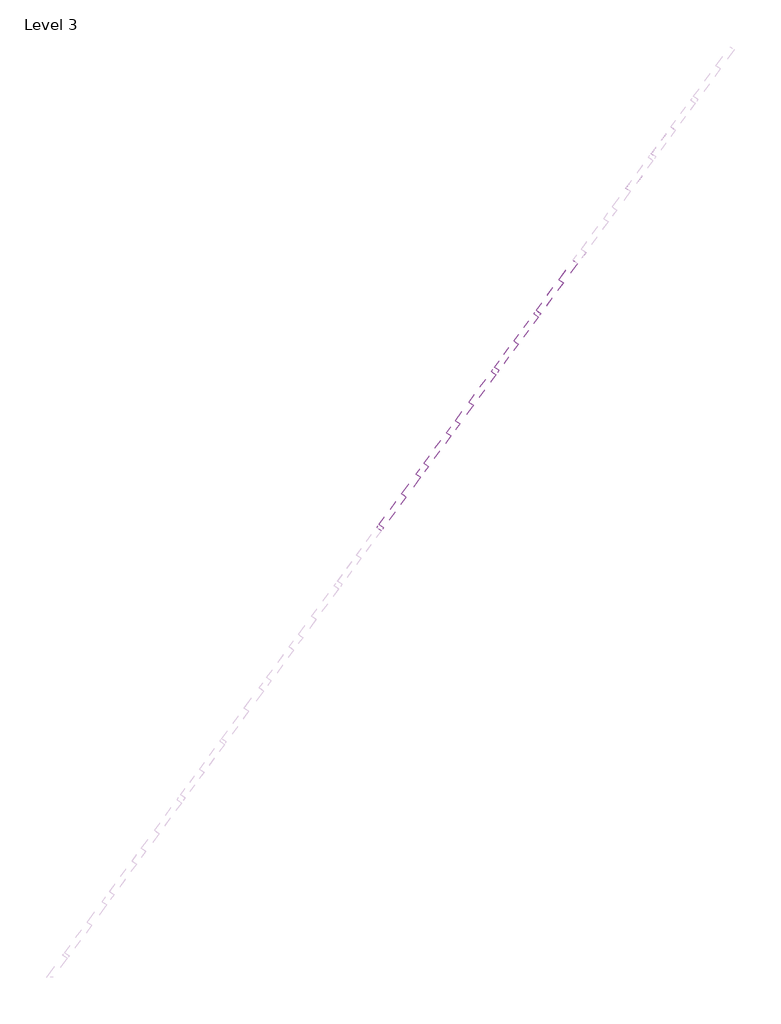
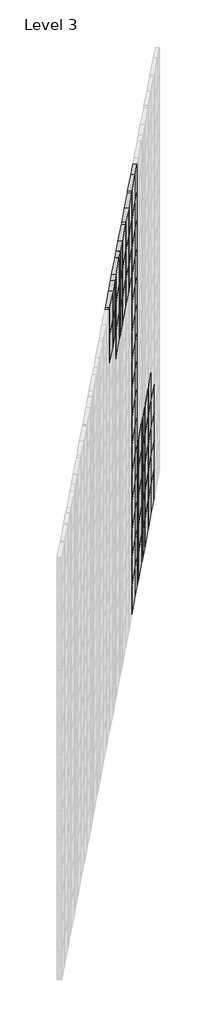
# One storey, part 8 of 9: 117 plates.
"""IFC4 building model written with IfcOpenShell, lengths in millimetres."""

import ifcopenshell
import ifcopenshell.guid

model = None  # the IFC model being written
_history = None  # IfcOwnerHistory: only IFC2X3 demands one
_inside = {}  # id of a spatial element -> (the spatial element, [elements in it])
_under = {}  # id of a project, library or spatial element -> (it, [spatial elements below it])
_declared = {}  # id of a project -> (the project, [libraries it declares])
_typed = {}  # id of a type object -> (the type object, [elements of that type])
_made_of = {}  # id of a material, layer set ... -> (it, [elements and type objects made of it])


def new_model(schema):
    """Start an empty IFC model of exactly this schema.

    Asked for "IFC4X3", IfcOpenShell would pick the latest addendum, in which some entities
    have other attributes; the version numbers below select the first issue.
    IFC2X3 requires an IfcOwnerHistory on every rooted entity: one is made here for all.
    """
    global model, _history
    if schema == "IFC4X3":
        model = ifcopenshell.file(schema_version=(4, 3, 0, 0))
    else:
        model = ifcopenshell.file(schema=schema)
    _inside.clear()
    _under.clear()
    _declared.clear()
    _typed.clear()
    _made_of.clear()
    _history = None
    if model.schema == "IFC2X3":
        org = make("IfcOrganization", Name="unknown")
        user = make(
            "IfcPersonAndOrganization",
            ThePerson=make("IfcPerson", FamilyName="unknown"),
            TheOrganization=org,
        )
        app = make(
            "IfcApplication",
            ApplicationDeveloper=org,
            Version="unknown",
            ApplicationFullName="unknown",
            ApplicationIdentifier="unknown",
        )
        _history = make(
            "IfcOwnerHistory",
            OwningUser=user,
            OwningApplication=app,
            ChangeAction="ADDED",
            CreationDate=0,
        )
    return model


def make(cls, **values):
    """One entity of the class cls with the attributes given. An attribute that is None is left unset."""
    return model.create_entity(
        cls, **{name: value for name, value in values.items() if value is not None}
    )


def rooted(cls, **values):
    """An entity with a GlobalId (a new one), such as an element, a storey or a relation."""
    return make(cls, GlobalId=ifcopenshell.guid.new(), OwnerHistory=_history, **values)


def si_unit(unit_type, name, prefix=None):
    """IfcSIUnit, for example si_unit("LENGTHUNIT", "METRE", prefix="MILLI")."""
    return make("IfcSIUnit", UnitType=unit_type, Prefix=prefix, Name=name)


def assignment(units):
    """IfcUnitAssignment: the units of a project."""
    return None if units is None else make("IfcUnitAssignment", Units=units)


def point(xyz):
    """IfcCartesianPoint."""
    return None if xyz is None else make("IfcCartesianPoint", Coordinates=xyz)


def direction(xyz):
    """IfcDirection."""
    return None if xyz is None else make("IfcDirection", DirectionRatios=xyz)


def frame(location, z_axis=None, x_axis=None):
    """IfcAxis2Placement3D, a coordinate frame: its origin and axes. An axis left out is left unset."""
    return make(
        "IfcAxis2Placement3D",
        Location=point(location),
        Axis=direction(z_axis),
        RefDirection=direction(x_axis),
    )


def origin():
    """The frame at (0, 0, 0) with its axes left unset."""
    return frame((0.0, 0.0, 0.0))


def origin_with_axes():
    """The frame at (0, 0, 0) with the z axis (0, 0, 1) and the x axis (1, 0, 0) written out."""
    return frame((0.0, 0.0, 0.0), z_axis=(0.0, 0.0, 1.0), x_axis=(1.0, 0.0, 0.0))


def place(relative_to, where):
    """IfcLocalPlacement: puts the frame where relative to a parent placement (None: the world)."""
    return make(
        "IfcLocalPlacement", PlacementRelTo=relative_to, RelativePlacement=where
    )


def context(
    kind, dimensions, precision=None, world=None, true_north=None, identifier=None
):
    """IfcGeometricRepresentationContext, for example the 3D "Model" context."""
    return make(
        "IfcGeometricRepresentationContext",
        ContextIdentifier=identifier,
        ContextType=kind,
        CoordinateSpaceDimension=dimensions,
        Precision=precision,
        WorldCoordinateSystem=world,
        TrueNorth=true_north,
    )


def project(units=None, contexts=None):
    """IfcProject with its units and contexts."""
    return rooted(
        "IfcProject",
        Name="project",
        RepresentationContexts=contexts,
        UnitsInContext=assignment(units),
    )


def spatial(cls, under=None, at=None, **own):
    """A site, building, storey or space (cls), placed at a placement, below another one or the project."""
    s = rooted(cls, ObjectPlacement=at, **own)
    if under is not None:
        _under.setdefault(under.id(), (under, []))[1].append(s)
    return s


def polyline(points):
    """IfcPolyline through the points."""
    return make("IfcPolyline", Points=[point(p) for p in points])


def outline(outer, holes=None, kind="AREA"):
    """IfcArbitraryClosedProfileDef: a profile drawn as a closed curve; with holes, ...WithVoids."""
    if holes is None:
        return make("IfcArbitraryClosedProfileDef", ProfileType=kind, OuterCurve=outer)
    return make(
        "IfcArbitraryProfileDefWithVoids",
        ProfileType=kind,
        OuterCurve=outer,
        InnerCurves=holes,
    )


def extrude(swept, where, along, depth):
    """IfcExtrudedAreaSolid: the profile swept, set in the frame where, extruded along a direction by depth."""
    return make(
        "IfcExtrudedAreaSolid",
        SweptArea=swept,
        Position=where,
        ExtrudedDirection=direction(along),
        Depth=depth,
    )


def shape(context_of_items, identifier, shape_type, items):
    """IfcShapeRepresentation: the items that make up one representation, for example the "Body"."""
    return make(
        "IfcShapeRepresentation",
        ContextOfItems=context_of_items,
        RepresentationIdentifier=identifier,
        RepresentationType=shape_type,
        Items=items,
    )


def source(mapping_origin, context_of_items, identifier, shape_type, items):
    """IfcRepresentationMap: a shape defined once, which mapped items show again and again."""
    return make(
        "IfcRepresentationMap",
        MappingOrigin=mapping_origin,
        MappedRepresentation=shape(context_of_items, identifier, shape_type, items),
    )


def transform(
    local_origin,
    x_axis=None,
    y_axis=None,
    z_axis=None,
    scale=None,
    scale2=None,
    scale3=None,
    uniform=True,
):
    """IfcCartesianTransformationOperator3D, or its non-uniform kind. x_axis, y_axis, z_axis: its Axis1, 2, 3."""
    if uniform:
        return make(
            "IfcCartesianTransformationOperator3D",
            Axis1=direction(x_axis),
            Axis2=direction(y_axis),
            LocalOrigin=point(local_origin),
            Scale=scale,
            Axis3=direction(z_axis),
        )
    return make(
        "IfcCartesianTransformationOperator3DnonUniform",
        Axis1=direction(x_axis),
        Axis2=direction(y_axis),
        LocalOrigin=point(local_origin),
        Scale=scale,
        Axis3=direction(z_axis),
        Scale2=scale2,
        Scale3=scale3,
    )


def mapped(mapping_source, mapping_target):
    """IfcMappedItem: shows the shape of a source again, moved by a transform."""
    return make(
        "IfcMappedItem", MappingSource=mapping_source, MappingTarget=mapping_target
    )


def made_of(thing, what):
    """Note that an element or type object is made of a material, layer set ...; save() writes the relation."""
    if what is not None:
        _made_of.setdefault(what.id(), (what, []))[1].append(thing)
    return thing


def element(
    cls,
    number,
    at=None,
    inside=None,
    cuts=None,
    type_object=None,
    material=None,
    context=None,
    identifier="Body",
    shape_type=None,
    held_by="IfcProductDefinitionShape",
    body=None,
    shapes=None,
    **own,
):
    """One element of the class cls, such as IfcWall. Its Tag is "e" and its number.

    at: its placement. inside: the storey or other place that contains it. cuts: it is an
    opening in that element (IfcRelVoidsElement). A single representation is given by context,
    identifier, shape_type and body (its items); several are given by shapes. held_by: the class
    of the entity that holds the representations. save() writes the other relations.
    """
    e = rooted(cls, Tag="e%d" % number, ObjectPlacement=at, **own)
    if body is not None:
        shapes = [shape(context, identifier, shape_type, body)]
    if shapes is not None:
        e.Representation = make(held_by, Representations=shapes)
    if inside is not None:
        _inside.setdefault(inside.id(), (inside, []))[1].append(e)
    if cuts is not None:
        rooted(
            "IfcRelVoidsElement", RelatingBuildingElement=cuts, RelatedOpeningElement=e
        )
    if type_object is not None:
        _typed.setdefault(type_object.id(), (type_object, []))[1].append(e)
    return made_of(e, material)


def aggregate(whole, parts):
    """IfcRelAggregates: a whole, such as a stair, and the parts it consists of."""
    return rooted("IfcRelAggregates", RelatingObject=whole, RelatedObjects=parts)


def save(model, path):
    """Write the relations noted so far, then the file.

    IfcRelAggregates (storeys below a building ...), IfcRelContainedInSpatialStructure (elements
    in a storey), IfcRelDefinesByType, IfcRelAssociatesMaterial and IfcRelDeclares: one each for
    every whole, place, type object, material and project.
    """
    for whole, parts in _under.values():
        aggregate(whole, parts)
    for where, things in _inside.values():
        rooted(
            "IfcRelContainedInSpatialStructure",
            RelatedElements=things,
            RelatingStructure=where,
        )
    for kind, things in _typed.values():
        rooted("IfcRelDefinesByType", RelatedObjects=things, RelatingType=kind)
    for what, things in _made_of.values():
        rooted("IfcRelAssociatesMaterial", RelatedObjects=things, RelatingMaterial=what)
    for by, libraries in _declared.values():
        rooted("IfcRelDeclares", RelatingContext=by, RelatedDefinitions=libraries)
    model.write(path)


def system_panel_glazed_b646d57f(model_context):
    return source(origin(), model_context, "Body", "SweptSolid", [
        extrude(outline(polyline([(8.5363468, 24.5), (-8.5363468, 24.5), (-8.5363468, 49.5), (8.5363468, 49.5), (8.5363468, 24.5)])), origin_with_axes(), (0.0, 0.0, 1.0), 200.0),
    ])


def system_panel_glazed_944c5575(model_context):
    return source(origin(), model_context, "Body", "SweptSolid", [
        extrude(outline(polyline([(30.0531077, 24.5), (-30.0531077, 24.5), (-30.0531077, 49.5), (30.0531077, 49.5), (30.0531077, 24.5)])), origin_with_axes(), (0.0, 0.0, 1.0), 200.0),
    ])


def system_panel_glazed_4b393385(model_context):
    return source(origin(), model_context, "Body", "SweptSolid", [
        extrude(outline(polyline([(51.5698685, 24.5), (-51.5698685, 24.5), (-51.5698685, 49.5), (51.5698685, 49.5), (51.5698685, 24.5)])), origin_with_axes(), (0.0, 0.0, 1.0), 200.0),
    ])


def system_panel_glazed_44cc28f0(model_context):
    return source(origin(), model_context, "Body", "SweptSolid", [
        extrude(outline(polyline([(73.0866293, 24.5), (-73.0866293, 24.5), (-73.0866293, 49.5), (73.0866293, 49.5), (73.0866293, 24.5)])), origin_with_axes(), (0.0, 0.0, 1.0), 200.0),
    ])


def system_panel_glazed_1102e745(model_context):
    return source(origin(), model_context, "Body", "SweptSolid", [
        extrude(outline(polyline([(9.6033902, 24.5), (-9.6033902, 24.5), (-9.6033902, 49.5), (9.6033902, 49.5), (9.6033902, 24.5)])), origin_with_axes(), (0.0, 0.0, 1.0), 200.0),
    ])


def system_panel_glazed_6880485c(model_context):
    return source(origin(), model_context, "Body", "SweptSolid", [
        extrude(outline(polyline([(31.120151, 24.5), (-31.120151, 24.5), (-31.120151, 49.5), (31.120151, 49.5), (31.120151, 24.5)])), origin_with_axes(), (0.0, 0.0, 1.0), 200.0),
    ])


def system_panel_glazed_65218e73(model_context):
    return source(origin(), model_context, "Body", "SweptSolid", [
        extrude(outline(polyline([(52.6369119, 24.5), (-52.6369119, 24.5), (-52.6369119, 49.5), (52.6369119, 49.5), (52.6369119, 24.5)])), origin_with_axes(), (0.0, 0.0, 1.0), 200.0),
    ])


def system_panel_glazed_2ba9a9ff(model_context):
    return source(origin(), model_context, "Body", "SweptSolid", [
        extrude(outline(polyline([(74.1536727, 24.5), (-74.1536727, 24.5), (-74.1536727, 49.5), (74.1536727, 49.5), (74.1536727, 24.5)])), origin_with_axes(), (0.0, 0.0, 1.0), 200.0),
    ])


def system_panel_glazed_87147500(model_context):
    return source(origin(), model_context, "Body", "SweptSolid", [
        extrude(outline(polyline([(10.6704335, 24.5), (-10.6704335, 24.5), (-10.6704335, 49.5), (10.6704335, 49.5), (10.6704335, 24.5)])), origin_with_axes(), (0.0, 0.0, 1.0), 200.0),
    ])


def system_panel_glazed_1ea8d406(model_context):
    return source(origin(), model_context, "Body", "SweptSolid", [
        extrude(outline(polyline([(85.0, 24.5), (-85.0, 24.5), (-85.0, 49.5), (85.0, 49.5), (85.0, 24.5)])), origin_with_axes(), (0.0, 0.0, 1.0), 200.0),
    ])


def system_panel_glazed_a6cffc9f(model_context):
    return source(origin(), model_context, "Body", "SweptSolid", [
        extrude(outline(polyline([(54.9468923, 24.5), (-54.9468923, 24.5), (-54.9468923, 49.5), (54.9468923, 49.5), (54.9468923, 24.5)])), origin_with_axes(), (0.0, 0.0, 1.0), 200.0),
    ])


def system_panel_glazed_52e3984b(model_context):
    return source(origin(), model_context, "Body", "SweptSolid", [
        extrude(outline(polyline([(33.4301315, 24.5), (-33.4301315, 24.5), (-33.4301315, 49.5), (33.4301315, 49.5), (33.4301315, 24.5)])), origin_with_axes(), (0.0, 0.0, 1.0), 200.0),
    ])


def system_panel_glazed_aeb916ba(model_context):
    return source(origin(), model_context, "Body", "SweptSolid", [
        extrude(outline(polyline([(11.9133707, 24.5), (-11.9133707, 24.5), (-11.9133707, 49.5), (11.9133707, 49.5), (11.9133707, 24.5)])), origin_with_axes(), (0.0, 0.0, 1.0), 200.0),
    ])


def system_panel_glazed_a3c9f580(model_context):
    return source(origin(), model_context, "Body", "SweptSolid", [
        extrude(outline(polyline([(75.3966098, 24.5), (-75.3966098, 24.5), (-75.3966098, 49.5), (75.3966098, 49.5), (75.3966098, 24.5)])), origin_with_axes(), (0.0, 0.0, 1.0), 200.0),
    ])


def system_panel_glazed_1c271f2e(model_context):
    return source(origin(), model_context, "Body", "SweptSolid", [
        extrude(outline(polyline([(53.879849, 24.5), (-53.879849, 24.5), (-53.879849, 49.5), (53.879849, 49.5), (53.879849, 24.5)])), origin_with_axes(), (0.0, 0.0, 1.0), 200.0),
    ])


def system_panel_glazed_d23853e5(model_context):
    return source(origin(), model_context, "Body", "SweptSolid", [
        extrude(outline(polyline([(32.3630881, 24.5), (-32.3630881, 24.5), (-32.3630881, 49.5), (32.3630881, 49.5), (32.3630881, 24.5)])), origin_with_axes(), (0.0, 0.0, 1.0), 200.0),
    ])


def system_panel_glazed_c2638314(model_context):
    return source(origin(), model_context, "Body", "SweptSolid", [
        extrude(outline(polyline([(10.8463273, 24.5), (-10.8463273, 24.5), (-10.8463273, 49.5), (10.8463273, 49.5), (10.8463273, 24.5)])), origin_with_axes(), (0.0, 0.0, 1.0), 200.0),
    ])


def system_panel_glazed_937a8ef3(model_context):
    return source(origin(), model_context, "Body", "SweptSolid", [
        extrude(outline(polyline([(74.3295665, 24.5), (-74.3295665, 24.5), (-74.3295665, 49.5), (74.3295665, 49.5), (74.3295665, 24.5)])), origin_with_axes(), (0.0, 0.0, 1.0), 200.0),
    ])


model = new_model("IFC4")

# Units and contexts
model_context = context("Model", 3, world=origin())
ifc_project = project(units=[si_unit("LENGTHUNIT", "METRE", prefix="MILLI")], contexts=[model_context])

# Site, building, storey
site = spatial("IfcSite", under=ifc_project)
building = spatial("IfcBuilding", under=site)
storey = spatial("IfcBuildingStorey", under=building, Name="Level 3", Elevation=22950.0)

# Plates
placement = place(None, origin())
system_panel_glazed_shape = system_panel_glazed_b646d57f(model_context)
element("IfcPlate", 1, ObjectType="System Panel : Glazed", at=placement, inside=storey, context=model_context, shape_type="MappedRepresentation", body=[
    mapped(system_panel_glazed_shape, transform((-31872.965562, 30068.174428, 37700.0), x_axis=(0.5920548138930122, 0.8058976965757569, 0.0), y_axis=(-0.8058976965757569, 0.5920548138930122, 0.0), z_axis=(0.0, 0.0, 1.0))),
])
element("IfcPlate", 2, ObjectType="System Panel : Glazed", at=placement, inside=storey, context=model_context, shape_type="MappedRepresentation", body=[
    mapped(system_panel_glazed_shape, transform((-31872.965562, 30068.174428, 37900.0), x_axis=(0.5920548138930122, 0.8058976965757569, 0.0), y_axis=(-0.8058976965757569, 0.5920548138930122, 0.0), z_axis=(0.0, 0.0, 1.0))),
])
system_panel_glazed_2_shape = system_panel_glazed_944c5575(model_context)
element("IfcPlate", 3, ObjectType="System Panel : Glazed", at=placement, inside=storey, context=model_context, shape_type="MappedRepresentation", body=[
    mapped(system_panel_glazed_2_shape, transform((-31684.4060271, 30324.8393368, 37700.0), x_axis=(0.5920548138930122, 0.8058976965757569, 0.0), y_axis=(-0.8058976965757569, 0.5920548138930122, 0.0), z_axis=(0.0, 0.0, 1.0))),
])
element("IfcPlate", 4, ObjectType="System Panel : Glazed", at=placement, inside=storey, context=model_context, shape_type="MappedRepresentation", body=[
    mapped(system_panel_glazed_2_shape, transform((-31684.4060271, 30324.8393368, 37900.0), x_axis=(0.5920548138930122, 0.8058976965757569, 0.0), y_axis=(-0.8058976965757569, 0.5920548138930122, 0.0), z_axis=(0.0, 0.0, 1.0))),
])
system_panel_glazed_3_shape = system_panel_glazed_4b393385(model_context)
element("IfcPlate", 5, ObjectType="System Panel : Glazed", at=placement, inside=storey, context=model_context, shape_type="MappedRepresentation", body=[
    mapped(system_panel_glazed_3_shape, transform((-31495.8464922, 30581.5042456, 37500.0), x_axis=(0.5920548138930122, 0.8058976965757569, 0.0), y_axis=(-0.8058976965757569, 0.5920548138930122, 0.0), z_axis=(0.0, 0.0, 1.0))),
])
element("IfcPlate", 6, ObjectType="System Panel : Glazed", at=placement, inside=storey, context=model_context, shape_type="MappedRepresentation", body=[
    mapped(system_panel_glazed_3_shape, transform((-31495.8464922, 30581.5042456, 37700.0), x_axis=(0.5920548138930122, 0.8058976965757569, 0.0), y_axis=(-0.8058976965757569, 0.5920548138930122, 0.0), z_axis=(0.0, 0.0, 1.0))),
])
element("IfcPlate", 7, ObjectType="System Panel : Glazed", at=placement, inside=storey, context=model_context, shape_type="MappedRepresentation", body=[
    mapped(system_panel_glazed_3_shape, transform((-31495.8464922, 30581.5042456, 37900.0), x_axis=(0.5920548138930122, 0.8058976965757569, 0.0), y_axis=(-0.8058976965757569, 0.5920548138930122, 0.0), z_axis=(0.0, 0.0, 1.0))),
])
system_panel_glazed_4_shape = system_panel_glazed_44cc28f0(model_context)
element("IfcPlate", 8, ObjectType="System Panel : Glazed", at=placement, inside=storey, context=model_context, shape_type="MappedRepresentation", body=[
    mapped(system_panel_glazed_4_shape, transform((-31307.2869573, 30838.1691545, 37500.0), x_axis=(0.5920548138930122, 0.8058976965757569, 0.0), y_axis=(-0.8058976965757569, 0.5920548138930122, 0.0), z_axis=(0.0, 0.0, 1.0))),
])
element("IfcPlate", 9, ObjectType="System Panel : Glazed", at=placement, inside=storey, context=model_context, shape_type="MappedRepresentation", body=[
    mapped(system_panel_glazed_4_shape, transform((-31307.2869573, 30838.1691545, 37700.0), x_axis=(0.5920548138930122, 0.8058976965757569, 0.0), y_axis=(-0.8058976965757569, 0.5920548138930122, 0.0), z_axis=(0.0, 0.0, 1.0))),
])
element("IfcPlate", 10, ObjectType="System Panel : Glazed", at=placement, inside=storey, context=model_context, shape_type="MappedRepresentation", body=[
    mapped(system_panel_glazed_4_shape, transform((-31307.2869573, 30838.1691545, 37900.0), x_axis=(0.5920548138930122, 0.8058976965757569, 0.0), y_axis=(-0.8058976965757569, 0.5920548138930122, 0.0), z_axis=(0.0, 0.0, 1.0))),
])
system_panel_glazed_5_shape = system_panel_glazed_1102e745(model_context)
element("IfcPlate", 11, ObjectType="System Panel : Glazed", at=placement, inside=storey, context=model_context, shape_type="MappedRepresentation", body=[
    mapped(system_panel_glazed_5_shape, transform((-31169.0520816, 31026.3327591, 35100.0), x_axis=(0.5920548138930122, 0.8058976965757569, 0.0), y_axis=(-0.8058976965757569, 0.5920548138930122, 0.0), z_axis=(0.0, 0.0, 1.0))),
])
element("IfcPlate", 12, ObjectType="System Panel : Glazed", at=placement, inside=storey, context=model_context, shape_type="MappedRepresentation", body=[
    mapped(system_panel_glazed_5_shape, transform((-31169.0520816, 31026.3327591, 35300.0), x_axis=(0.5920548138930122, 0.8058976965757569, 0.0), y_axis=(-0.8058976965757569, 0.5920548138930122, 0.0), z_axis=(0.0, 0.0, 1.0))),
])
element("IfcPlate", 13, ObjectType="System Panel : Glazed", at=placement, inside=storey, context=model_context, shape_type="MappedRepresentation", body=[
    mapped(system_panel_glazed_5_shape, transform((-31169.0520816, 31026.3327591, 35500.0), x_axis=(0.5920548138930122, 0.8058976965757569, 0.0), y_axis=(-0.8058976965757569, 0.5920548138930122, 0.0), z_axis=(0.0, 0.0, 1.0))),
])
element("IfcPlate", 14, ObjectType="System Panel : Glazed", at=placement, inside=storey, context=model_context, shape_type="MappedRepresentation", body=[
    mapped(system_panel_glazed_5_shape, transform((-31169.0520816, 31026.3327591, 35700.0), x_axis=(0.5920548138930122, 0.8058976965757569, 0.0), y_axis=(-0.8058976965757569, 0.5920548138930122, 0.0), z_axis=(0.0, 0.0, 1.0))),
])
element("IfcPlate", 15, ObjectType="System Panel : Glazed", at=placement, inside=storey, context=model_context, shape_type="MappedRepresentation", body=[
    mapped(system_panel_glazed_5_shape, transform((-31169.0520816, 31026.3327591, 35900.0), x_axis=(0.5920548138930122, 0.8058976965757569, 0.0), y_axis=(-0.8058976965757569, 0.5920548138930122, 0.0), z_axis=(0.0, 0.0, 1.0))),
])
element("IfcPlate", 16, ObjectType="System Panel : Glazed", at=placement, inside=storey, context=model_context, shape_type="MappedRepresentation", body=[
    mapped(system_panel_glazed_5_shape, transform((-31169.0520816, 31026.3327591, 36100.0), x_axis=(0.5920548138930122, 0.8058976965757569, 0.0), y_axis=(-0.8058976965757569, 0.5920548138930122, 0.0), z_axis=(0.0, 0.0, 1.0))),
])
element("IfcPlate", 17, ObjectType="System Panel : Glazed", at=placement, inside=storey, context=model_context, shape_type="MappedRepresentation", body=[
    mapped(system_panel_glazed_5_shape, transform((-31169.0520816, 31026.3327591, 36300.0), x_axis=(0.5920548138930122, 0.8058976965757569, 0.0), y_axis=(-0.8058976965757569, 0.5920548138930122, 0.0), z_axis=(0.0, 0.0, 1.0))),
])
element("IfcPlate", 18, ObjectType="System Panel : Glazed", at=placement, inside=storey, context=model_context, shape_type="MappedRepresentation", body=[
    mapped(system_panel_glazed_5_shape, transform((-31169.0520816, 31026.3327591, 36500.0), x_axis=(0.5920548138930122, 0.8058976965757569, 0.0), y_axis=(-0.8058976965757569, 0.5920548138930122, 0.0), z_axis=(0.0, 0.0, 1.0))),
])
element("IfcPlate", 19, ObjectType="System Panel : Glazed", at=placement, inside=storey, context=model_context, shape_type="MappedRepresentation", body=[
    mapped(system_panel_glazed_5_shape, transform((-31169.0520816, 31026.3327591, 36700.0), x_axis=(0.5920548138930122, 0.8058976965757569, 0.0), y_axis=(-0.8058976965757569, 0.5920548138930122, 0.0), z_axis=(0.0, 0.0, 1.0))),
])
element("IfcPlate", 20, ObjectType="System Panel : Glazed", at=placement, inside=storey, context=model_context, shape_type="MappedRepresentation", body=[
    mapped(system_panel_glazed_5_shape, transform((-31169.0520816, 31026.3327591, 36900.0), x_axis=(0.5920548138930122, 0.8058976965757569, 0.0), y_axis=(-0.8058976965757569, 0.5920548138930122, 0.0), z_axis=(0.0, 0.0, 1.0))),
])
element("IfcPlate", 21, ObjectType="System Panel : Glazed", at=placement, inside=storey, context=model_context, shape_type="MappedRepresentation", body=[
    mapped(system_panel_glazed_5_shape, transform((-31169.0520816, 31026.3327591, 37100.0), x_axis=(0.5920548138930122, 0.8058976965757569, 0.0), y_axis=(-0.8058976965757569, 0.5920548138930122, 0.0), z_axis=(0.0, 0.0, 1.0))),
])
element("IfcPlate", 22, ObjectType="System Panel : Glazed", at=placement, inside=storey, context=model_context, shape_type="MappedRepresentation", body=[
    mapped(system_panel_glazed_5_shape, transform((-31169.0520816, 31026.3327591, 37300.0), x_axis=(0.5920548138930122, 0.8058976965757569, 0.0), y_axis=(-0.8058976965757569, 0.5920548138930122, 0.0), z_axis=(0.0, 0.0, 1.0))),
])
element("IfcPlate", 23, ObjectType="System Panel : Glazed", at=placement, inside=storey, context=model_context, shape_type="MappedRepresentation", body=[
    mapped(system_panel_glazed_5_shape, transform((-31169.0520816, 31026.3327591, 37500.0), x_axis=(0.5920548138930122, 0.8058976965757569, 0.0), y_axis=(-0.8058976965757569, 0.5920548138930122, 0.0), z_axis=(0.0, 0.0, 1.0))),
])
element("IfcPlate", 24, ObjectType="System Panel : Glazed", at=placement, inside=storey, context=model_context, shape_type="MappedRepresentation", body=[
    mapped(system_panel_glazed_5_shape, transform((-31169.0520816, 31026.3327591, 37700.0), x_axis=(0.5920548138930122, 0.8058976965757569, 0.0), y_axis=(-0.8058976965757569, 0.5920548138930122, 0.0), z_axis=(0.0, 0.0, 1.0))),
])
element("IfcPlate", 25, ObjectType="System Panel : Glazed", at=placement, inside=storey, context=model_context, shape_type="MappedRepresentation", body=[
    mapped(system_panel_glazed_5_shape, transform((-31169.0520816, 31026.3327591, 37900.0), x_axis=(0.5920548138930122, 0.8058976965757569, 0.0), y_axis=(-0.8058976965757569, 0.5920548138930122, 0.0), z_axis=(0.0, 0.0, 1.0))),
])
system_panel_glazed_6_shape = system_panel_glazed_6880485c(model_context)
element("IfcPlate", 26, ObjectType="System Panel : Glazed", at=placement, inside=storey, context=model_context, shape_type="MappedRepresentation", body=[
    mapped(system_panel_glazed_6_shape, transform((-30980.4925467, 31282.997668, 35100.0), x_axis=(0.5920548138930122, 0.8058976965757569, 0.0), y_axis=(-0.8058976965757569, 0.5920548138930122, 0.0), z_axis=(0.0, 0.0, 1.0))),
])
element("IfcPlate", 27, ObjectType="System Panel : Glazed", at=placement, inside=storey, context=model_context, shape_type="MappedRepresentation", body=[
    mapped(system_panel_glazed_6_shape, transform((-30980.4925467, 31282.997668, 35300.0), x_axis=(0.5920548138930122, 0.8058976965757569, 0.0), y_axis=(-0.8058976965757569, 0.5920548138930122, 0.0), z_axis=(0.0, 0.0, 1.0))),
])
element("IfcPlate", 28, ObjectType="System Panel : Glazed", at=placement, inside=storey, context=model_context, shape_type="MappedRepresentation", body=[
    mapped(system_panel_glazed_6_shape, transform((-30980.4925467, 31282.997668, 35500.0), x_axis=(0.5920548138930122, 0.8058976965757569, 0.0), y_axis=(-0.8058976965757569, 0.5920548138930122, 0.0), z_axis=(0.0, 0.0, 1.0))),
])
element("IfcPlate", 29, ObjectType="System Panel : Glazed", at=placement, inside=storey, context=model_context, shape_type="MappedRepresentation", body=[
    mapped(system_panel_glazed_6_shape, transform((-30980.4925467, 31282.997668, 35700.0), x_axis=(0.5920548138930122, 0.8058976965757569, 0.0), y_axis=(-0.8058976965757569, 0.5920548138930122, 0.0), z_axis=(0.0, 0.0, 1.0))),
])
element("IfcPlate", 30, ObjectType="System Panel : Glazed", at=placement, inside=storey, context=model_context, shape_type="MappedRepresentation", body=[
    mapped(system_panel_glazed_6_shape, transform((-30980.4925467, 31282.997668, 35900.0), x_axis=(0.5920548138930122, 0.8058976965757569, 0.0), y_axis=(-0.8058976965757569, 0.5920548138930122, 0.0), z_axis=(0.0, 0.0, 1.0))),
])
system_panel_glazed_7_shape = system_panel_glazed_65218e73(model_context)
element("IfcPlate", 31, ObjectType="System Panel : Glazed", at=placement, inside=storey, context=model_context, shape_type="MappedRepresentation", body=[
    mapped(system_panel_glazed_7_shape, transform((-30791.9330118, 31539.6625768, 35100.0), x_axis=(0.5920548138930122, 0.8058976965757569, 0.0), y_axis=(-0.8058976965757569, 0.5920548138930122, 0.0), z_axis=(0.0, 0.0, 1.0))),
])
element("IfcPlate", 32, ObjectType="System Panel : Glazed", at=placement, inside=storey, context=model_context, shape_type="MappedRepresentation", body=[
    mapped(system_panel_glazed_7_shape, transform((-30791.9330118, 31539.6625768, 35300.0), x_axis=(0.5920548138930122, 0.8058976965757569, 0.0), y_axis=(-0.8058976965757569, 0.5920548138930122, 0.0), z_axis=(0.0, 0.0, 1.0))),
])
element("IfcPlate", 33, ObjectType="System Panel : Glazed", at=placement, inside=storey, context=model_context, shape_type="MappedRepresentation", body=[
    mapped(system_panel_glazed_7_shape, transform((-30791.9330118, 31539.6625768, 35500.0), x_axis=(0.5920548138930122, 0.8058976965757569, 0.0), y_axis=(-0.8058976965757569, 0.5920548138930122, 0.0), z_axis=(0.0, 0.0, 1.0))),
])
element("IfcPlate", 34, ObjectType="System Panel : Glazed", at=placement, inside=storey, context=model_context, shape_type="MappedRepresentation", body=[
    mapped(system_panel_glazed_7_shape, transform((-30791.9330118, 31539.6625768, 35700.0), x_axis=(0.5920548138930122, 0.8058976965757569, 0.0), y_axis=(-0.8058976965757569, 0.5920548138930122, 0.0), z_axis=(0.0, 0.0, 1.0))),
])
element("IfcPlate", 35, ObjectType="System Panel : Glazed", at=placement, inside=storey, context=model_context, shape_type="MappedRepresentation", body=[
    mapped(system_panel_glazed_7_shape, transform((-30791.9330118, 31539.6625768, 35900.0), x_axis=(0.5920548138930122, 0.8058976965757569, 0.0), y_axis=(-0.8058976965757569, 0.5920548138930122, 0.0), z_axis=(0.0, 0.0, 1.0))),
])
system_panel_glazed_8_shape = system_panel_glazed_2ba9a9ff(model_context)
element("IfcPlate", 36, ObjectType="System Panel : Glazed", at=placement, inside=storey, context=model_context, shape_type="MappedRepresentation", body=[
    mapped(system_panel_glazed_8_shape, transform((-30603.373477, 31796.3274856, 35100.0), x_axis=(0.5920548138930122, 0.8058976965757569, 0.0), y_axis=(-0.8058976965757569, 0.5920548138930122, 0.0), z_axis=(0.0, 0.0, 1.0))),
])
element("IfcPlate", 37, ObjectType="System Panel : Glazed", at=placement, inside=storey, context=model_context, shape_type="MappedRepresentation", body=[
    mapped(system_panel_glazed_8_shape, transform((-30603.373477, 31796.3274856, 35300.0), x_axis=(0.5920548138930122, 0.8058976965757569, 0.0), y_axis=(-0.8058976965757569, 0.5920548138930122, 0.0), z_axis=(0.0, 0.0, 1.0))),
])
element("IfcPlate", 38, ObjectType="System Panel : Glazed", at=placement, inside=storey, context=model_context, shape_type="MappedRepresentation", body=[
    mapped(system_panel_glazed_8_shape, transform((-30603.373477, 31796.3274856, 35500.0), x_axis=(0.5920548138930122, 0.8058976965757569, 0.0), y_axis=(-0.8058976965757569, 0.5920548138930122, 0.0), z_axis=(0.0, 0.0, 1.0))),
])
element("IfcPlate", 39, ObjectType="System Panel : Glazed", at=placement, inside=storey, context=model_context, shape_type="MappedRepresentation", body=[
    mapped(system_panel_glazed_8_shape, transform((-30603.373477, 31796.3274856, 35700.0), x_axis=(0.5920548138930122, 0.8058976965757569, 0.0), y_axis=(-0.8058976965757569, 0.5920548138930122, 0.0), z_axis=(0.0, 0.0, 1.0))),
])
element("IfcPlate", 40, ObjectType="System Panel : Glazed", at=placement, inside=storey, context=model_context, shape_type="MappedRepresentation", body=[
    mapped(system_panel_glazed_8_shape, transform((-30603.373477, 31796.3274856, 35900.0), x_axis=(0.5920548138930122, 0.8058976965757569, 0.0), y_axis=(-0.8058976965757569, 0.5920548138930122, 0.0), z_axis=(0.0, 0.0, 1.0))),
])
system_panel_glazed_9_shape = system_panel_glazed_87147500(model_context)
element("IfcPlate", 41, ObjectType="System Panel : Glazed", at=placement, inside=storey, context=model_context, shape_type="MappedRepresentation", body=[
    mapped(system_panel_glazed_9_shape, transform((-30465.1386012, 31984.4910903, 35100.0), x_axis=(0.5920548138930122, 0.8058976965757569, 0.0), y_axis=(-0.8058976965757569, 0.5920548138930122, 0.0), z_axis=(0.0, 0.0, 1.0))),
])
element("IfcPlate", 42, ObjectType="System Panel : Glazed", at=placement, inside=storey, context=model_context, shape_type="MappedRepresentation", body=[
    mapped(system_panel_glazed_9_shape, transform((-30465.1386012, 31984.4910903, 35300.0), x_axis=(0.5920548138930122, 0.8058976965757569, 0.0), y_axis=(-0.8058976965757569, 0.5920548138930122, 0.0), z_axis=(0.0, 0.0, 1.0))),
])
element("IfcPlate", 43, ObjectType="System Panel : Glazed", at=placement, inside=storey, context=model_context, shape_type="MappedRepresentation", body=[
    mapped(system_panel_glazed_9_shape, transform((-30465.1386012, 31984.4910903, 35500.0), x_axis=(0.5920548138930122, 0.8058976965757569, 0.0), y_axis=(-0.8058976965757569, 0.5920548138930122, 0.0), z_axis=(0.0, 0.0, 1.0))),
])
element("IfcPlate", 44, ObjectType="System Panel : Glazed", at=placement, inside=storey, context=model_context, shape_type="MappedRepresentation", body=[
    mapped(system_panel_glazed_9_shape, transform((-30465.1386012, 31984.4910903, 35700.0), x_axis=(0.5920548138930122, 0.8058976965757569, 0.0), y_axis=(-0.8058976965757569, 0.5920548138930122, 0.0), z_axis=(0.0, 0.0, 1.0))),
])
system_panel_glazed_10_shape = system_panel_glazed_1ea8d406(model_context)
element("IfcPlate", 45, ObjectType="System Panel : Glazed", at=placement, inside=storey, context=model_context, shape_type="MappedRepresentation", body=[
    mapped(system_panel_glazed_10_shape, transform((-31113.0416891, 31102.5734133, 35100.0), x_axis=(0.5920548138930122, 0.8058976965757569, 0.0), y_axis=(-0.8058976965757569, 0.5920548138930122, 0.0), z_axis=(0.0, 0.0, 1.0))),
])
element("IfcPlate", 46, ObjectType="System Panel : Glazed", at=placement, inside=storey, context=model_context, shape_type="MappedRepresentation", body=[
    mapped(system_panel_glazed_10_shape, transform((-30911.7430523, 31376.5786302, 35100.0), x_axis=(0.5920548138930122, 0.8058976965757569, 0.0), y_axis=(-0.8058976965757569, 0.5920548138930122, 0.0), z_axis=(0.0, 0.0, 1.0))),
])
element("IfcPlate", 47, ObjectType="System Panel : Glazed", at=placement, inside=storey, context=model_context, shape_type="MappedRepresentation", body=[
    mapped(system_panel_glazed_10_shape, transform((-30710.4444156, 31650.583847, 35100.0), x_axis=(0.5920548138930122, 0.8058976965757569, 0.0), y_axis=(-0.8058976965757569, 0.5920548138930122, 0.0), z_axis=(0.0, 0.0, 1.0))),
])
element("IfcPlate", 48, ObjectType="System Panel : Glazed", at=placement, inside=storey, context=model_context, shape_type="MappedRepresentation", body=[
    mapped(system_panel_glazed_10_shape, transform((-31113.0416891, 31102.5734133, 35300.0), x_axis=(0.5920548138930122, 0.8058976965757569, 0.0), y_axis=(-0.8058976965757569, 0.5920548138930122, 0.0), z_axis=(0.0, 0.0, 1.0))),
])
element("IfcPlate", 49, ObjectType="System Panel : Glazed", at=placement, inside=storey, context=model_context, shape_type="MappedRepresentation", body=[
    mapped(system_panel_glazed_10_shape, transform((-30911.7430523, 31376.5786302, 35300.0), x_axis=(0.5920548138930122, 0.8058976965757569, 0.0), y_axis=(-0.8058976965757569, 0.5920548138930122, 0.0), z_axis=(0.0, 0.0, 1.0))),
])
element("IfcPlate", 50, ObjectType="System Panel : Glazed", at=placement, inside=storey, context=model_context, shape_type="MappedRepresentation", body=[
    mapped(system_panel_glazed_10_shape, transform((-30710.4444156, 31650.583847, 35300.0), x_axis=(0.5920548138930122, 0.8058976965757569, 0.0), y_axis=(-0.8058976965757569, 0.5920548138930122, 0.0), z_axis=(0.0, 0.0, 1.0))),
])
element("IfcPlate", 51, ObjectType="System Panel : Glazed", at=placement, inside=storey, context=model_context, shape_type="MappedRepresentation", body=[
    mapped(system_panel_glazed_10_shape, transform((-31113.0416891, 31102.5734133, 35500.0), x_axis=(0.5920548138930122, 0.8058976965757569, 0.0), y_axis=(-0.8058976965757569, 0.5920548138930122, 0.0), z_axis=(0.0, 0.0, 1.0))),
])
element("IfcPlate", 52, ObjectType="System Panel : Glazed", at=placement, inside=storey, context=model_context, shape_type="MappedRepresentation", body=[
    mapped(system_panel_glazed_10_shape, transform((-30911.7430523, 31376.5786302, 35500.0), x_axis=(0.5920548138930122, 0.8058976965757569, 0.0), y_axis=(-0.8058976965757569, 0.5920548138930122, 0.0), z_axis=(0.0, 0.0, 1.0))),
])
element("IfcPlate", 53, ObjectType="System Panel : Glazed", at=placement, inside=storey, context=model_context, shape_type="MappedRepresentation", body=[
    mapped(system_panel_glazed_10_shape, transform((-30710.4444156, 31650.583847, 35500.0), x_axis=(0.5920548138930122, 0.8058976965757569, 0.0), y_axis=(-0.8058976965757569, 0.5920548138930122, 0.0), z_axis=(0.0, 0.0, 1.0))),
])
element("IfcPlate", 54, ObjectType="System Panel : Glazed", at=placement, inside=storey, context=model_context, shape_type="MappedRepresentation", body=[
    mapped(system_panel_glazed_10_shape, transform((-31113.0416891, 31102.5734133, 35700.0), x_axis=(0.5920548138930122, 0.8058976965757569, 0.0), y_axis=(-0.8058976965757569, 0.5920548138930122, 0.0), z_axis=(0.0, 0.0, 1.0))),
])
element("IfcPlate", 55, ObjectType="System Panel : Glazed", at=placement, inside=storey, context=model_context, shape_type="MappedRepresentation", body=[
    mapped(system_panel_glazed_10_shape, transform((-30911.7430523, 31376.5786302, 35700.0), x_axis=(0.5920548138930122, 0.8058976965757569, 0.0), y_axis=(-0.8058976965757569, 0.5920548138930122, 0.0), z_axis=(0.0, 0.0, 1.0))),
])
element("IfcPlate", 56, ObjectType="System Panel : Glazed", at=placement, inside=storey, context=model_context, shape_type="MappedRepresentation", body=[
    mapped(system_panel_glazed_10_shape, transform((-30710.4444156, 31650.583847, 35700.0), x_axis=(0.5920548138930122, 0.8058976965757569, 0.0), y_axis=(-0.8058976965757569, 0.5920548138930122, 0.0), z_axis=(0.0, 0.0, 1.0))),
])
element("IfcPlate", 57, ObjectType="System Panel : Glazed", at=placement, inside=storey, context=model_context, shape_type="MappedRepresentation", body=[
    mapped(system_panel_glazed_10_shape, transform((-31113.0416891, 31102.5734133, 35900.0), x_axis=(0.5920548138930122, 0.8058976965757569, 0.0), y_axis=(-0.8058976965757569, 0.5920548138930122, 0.0), z_axis=(0.0, 0.0, 1.0))),
])
element("IfcPlate", 58, ObjectType="System Panel : Glazed", at=placement, inside=storey, context=model_context, shape_type="MappedRepresentation", body=[
    mapped(system_panel_glazed_10_shape, transform((-30911.7430523, 31376.5786302, 35900.0), x_axis=(0.5920548138930122, 0.8058976965757569, 0.0), y_axis=(-0.8058976965757569, 0.5920548138930122, 0.0), z_axis=(0.0, 0.0, 1.0))),
])
element("IfcPlate", 59, ObjectType="System Panel : Glazed", at=placement, inside=storey, context=model_context, shape_type="MappedRepresentation", body=[
    mapped(system_panel_glazed_10_shape, transform((-30710.4444156, 31650.583847, 35900.0), x_axis=(0.5920548138930122, 0.8058976965757569, 0.0), y_axis=(-0.8058976965757569, 0.5920548138930122, 0.0), z_axis=(0.0, 0.0, 1.0))),
])
element("IfcPlate", 60, ObjectType="System Panel : Glazed", at=placement, inside=storey, context=model_context, shape_type="MappedRepresentation", body=[
    mapped(system_panel_glazed_10_shape, transform((-31113.0416891, 31102.5734133, 36100.0), x_axis=(0.5920548138930122, 0.8058976965757569, 0.0), y_axis=(-0.8058976965757569, 0.5920548138930122, 0.0), z_axis=(0.0, 0.0, 1.0))),
])
element("IfcPlate", 61, ObjectType="System Panel : Glazed", at=placement, inside=storey, context=model_context, shape_type="MappedRepresentation", body=[
    mapped(system_panel_glazed_10_shape, transform((-31113.0416891, 31102.5734133, 36300.0), x_axis=(0.5920548138930122, 0.8058976965757569, 0.0), y_axis=(-0.8058976965757569, 0.5920548138930122, 0.0), z_axis=(0.0, 0.0, 1.0))),
])
element("IfcPlate", 62, ObjectType="System Panel : Glazed", at=placement, inside=storey, context=model_context, shape_type="MappedRepresentation", body=[
    mapped(system_panel_glazed_10_shape, transform((-31113.0416891, 31102.5734133, 36500.0), x_axis=(0.5920548138930122, 0.8058976965757569, 0.0), y_axis=(-0.8058976965757569, 0.5920548138930122, 0.0), z_axis=(0.0, 0.0, 1.0))),
])
element("IfcPlate", 63, ObjectType="System Panel : Glazed", at=placement, inside=storey, context=model_context, shape_type="MappedRepresentation", body=[
    mapped(system_panel_glazed_10_shape, transform((-31113.0416891, 31102.5734133, 36700.0), x_axis=(0.5920548138930122, 0.8058976965757569, 0.0), y_axis=(-0.8058976965757569, 0.5920548138930122, 0.0), z_axis=(0.0, 0.0, 1.0))),
])
element("IfcPlate", 64, ObjectType="System Panel : Glazed", at=placement, inside=storey, context=model_context, shape_type="MappedRepresentation", body=[
    mapped(system_panel_glazed_10_shape, transform((-31113.0416891, 31102.5734133, 36900.0), x_axis=(0.5920548138930122, 0.8058976965757569, 0.0), y_axis=(-0.8058976965757569, 0.5920548138930122, 0.0), z_axis=(0.0, 0.0, 1.0))),
])
element("IfcPlate", 65, ObjectType="System Panel : Glazed", at=placement, inside=storey, context=model_context, shape_type="MappedRepresentation", body=[
    mapped(system_panel_glazed_10_shape, transform((-31113.0416891, 31102.5734133, 37100.0), x_axis=(0.5920548138930122, 0.8058976965757569, 0.0), y_axis=(-0.8058976965757569, 0.5920548138930122, 0.0), z_axis=(0.0, 0.0, 1.0))),
])
element("IfcPlate", 66, ObjectType="System Panel : Glazed", at=placement, inside=storey, context=model_context, shape_type="MappedRepresentation", body=[
    mapped(system_panel_glazed_10_shape, transform((-31113.0416891, 31102.5734133, 37300.0), x_axis=(0.5920548138930122, 0.8058976965757569, 0.0), y_axis=(-0.8058976965757569, 0.5920548138930122, 0.0), z_axis=(0.0, 0.0, 1.0))),
])
element("IfcPlate", 67, ObjectType="System Panel : Glazed", at=placement, inside=storey, context=model_context, shape_type="MappedRepresentation", body=[
    mapped(system_panel_glazed_10_shape, transform((-31616.2882809, 30417.5603713, 37500.0), x_axis=(0.5920548138930122, 0.8058976965757569, 0.0), y_axis=(-0.8058976965757569, 0.5920548138930122, 0.0), z_axis=(0.0, 0.0, 1.0))),
])
element("IfcPlate", 68, ObjectType="System Panel : Glazed", at=placement, inside=storey, context=model_context, shape_type="MappedRepresentation", body=[
    mapped(system_panel_glazed_10_shape, transform((-31414.9896441, 30691.5655881, 37500.0), x_axis=(0.5920548138930122, 0.8058976965757569, 0.0), y_axis=(-0.8058976965757569, 0.5920548138930122, 0.0), z_axis=(0.0, 0.0, 1.0))),
])
element("IfcPlate", 69, ObjectType="System Panel : Glazed", at=placement, inside=storey, context=model_context, shape_type="MappedRepresentation", body=[
    mapped(system_panel_glazed_10_shape, transform((-31113.0416891, 31102.5734133, 37500.0), x_axis=(0.5920548138930122, 0.8058976965757569, 0.0), y_axis=(-0.8058976965757569, 0.5920548138930122, 0.0), z_axis=(0.0, 0.0, 1.0))),
])
element("IfcPlate", 70, ObjectType="System Panel : Glazed", at=placement, inside=storey, context=model_context, shape_type="MappedRepresentation", body=[
    mapped(system_panel_glazed_10_shape, transform((-31817.5869176, 30143.5551544, 37700.0), x_axis=(0.5920548138930122, 0.8058976965757569, 0.0), y_axis=(-0.8058976965757569, 0.5920548138930122, 0.0), z_axis=(0.0, 0.0, 1.0))),
])
element("IfcPlate", 71, ObjectType="System Panel : Glazed", at=placement, inside=storey, context=model_context, shape_type="MappedRepresentation", body=[
    mapped(system_panel_glazed_10_shape, transform((-31616.2882809, 30417.5603713, 37700.0), x_axis=(0.5920548138930122, 0.8058976965757569, 0.0), y_axis=(-0.8058976965757569, 0.5920548138930122, 0.0), z_axis=(0.0, 0.0, 1.0))),
])
element("IfcPlate", 72, ObjectType="System Panel : Glazed", at=placement, inside=storey, context=model_context, shape_type="MappedRepresentation", body=[
    mapped(system_panel_glazed_10_shape, transform((-31414.9896441, 30691.5655881, 37700.0), x_axis=(0.5920548138930122, 0.8058976965757569, 0.0), y_axis=(-0.8058976965757569, 0.5920548138930122, 0.0), z_axis=(0.0, 0.0, 1.0))),
])
element("IfcPlate", 73, ObjectType="System Panel : Glazed", at=placement, inside=storey, context=model_context, shape_type="MappedRepresentation", body=[
    mapped(system_panel_glazed_10_shape, transform((-31113.0416891, 31102.5734133, 37700.0), x_axis=(0.5920548138930122, 0.8058976965757569, 0.0), y_axis=(-0.8058976965757569, 0.5920548138930122, 0.0), z_axis=(0.0, 0.0, 1.0))),
])
element("IfcPlate", 74, ObjectType="System Panel : Glazed", at=placement, inside=storey, context=model_context, shape_type="MappedRepresentation", body=[
    mapped(system_panel_glazed_10_shape, transform((-31817.5869176, 30143.5551544, 37900.0), x_axis=(0.5920548138930122, 0.8058976965757569, 0.0), y_axis=(-0.8058976965757569, 0.5920548138930122, 0.0), z_axis=(0.0, 0.0, 1.0))),
])
element("IfcPlate", 75, ObjectType="System Panel : Glazed", at=placement, inside=storey, context=model_context, shape_type="MappedRepresentation", body=[
    mapped(system_panel_glazed_10_shape, transform((-31616.2882809, 30417.5603713, 37900.0), x_axis=(0.5920548138930122, 0.8058976965757569, 0.0), y_axis=(-0.8058976965757569, 0.5920548138930122, 0.0), z_axis=(0.0, 0.0, 1.0))),
])
element("IfcPlate", 76, ObjectType="System Panel : Glazed", at=placement, inside=storey, context=model_context, shape_type="MappedRepresentation", body=[
    mapped(system_panel_glazed_10_shape, transform((-31414.9896441, 30691.5655881, 37900.0), x_axis=(0.5920548138930122, 0.8058976965757569, 0.0), y_axis=(-0.8058976965757569, 0.5920548138930122, 0.0), z_axis=(0.0, 0.0, 1.0))),
])
element("IfcPlate", 77, ObjectType="System Panel : Glazed", at=placement, inside=storey, context=model_context, shape_type="MappedRepresentation", body=[
    mapped(system_panel_glazed_10_shape, transform((-31113.0416891, 31102.5734133, 37900.0), x_axis=(0.5920548138930122, 0.8058976965757569, 0.0), y_axis=(-0.8058976965757569, 0.5920548138930122, 0.0), z_axis=(0.0, 0.0, 1.0))),
])
system_panel_glazed_11_shape = system_panel_glazed_a6cffc9f(model_context)
element("IfcPlate", 78, ObjectType="System Panel : Glazed", at=placement, inside=storey, context=model_context, shape_type="MappedRepresentation", body=[
    mapped(system_panel_glazed_11_shape, transform((-31734.7306863, 30256.3380326, 37700.0), x_axis=(0.5920548138930122, 0.8058976965757569, 0.0), y_axis=(-0.8058976965757569, 0.5920548138930122, 0.0), z_axis=(0.0, 0.0, 1.0))),
])
element("IfcPlate", 79, ObjectType="System Panel : Glazed", at=placement, inside=storey, context=model_context, shape_type="MappedRepresentation", body=[
    mapped(system_panel_glazed_11_shape, transform((-31734.7306863, 30256.3380326, 37900.0), x_axis=(0.5920548138930122, 0.8058976965757569, 0.0), y_axis=(-0.8058976965757569, 0.5920548138930122, 0.0), z_axis=(0.0, 0.0, 1.0))),
])
system_panel_glazed_12_shape = system_panel_glazed_52e3984b(model_context)
element("IfcPlate", 80, ObjectType="System Panel : Glazed", at=placement, inside=storey, context=model_context, shape_type="MappedRepresentation", body=[
    mapped(system_panel_glazed_12_shape, transform((-31546.1711514, 30513.0029414, 37500.0), x_axis=(0.5920548138930122, 0.8058976965757569, 0.0), y_axis=(-0.8058976965757569, 0.5920548138930122, 0.0), z_axis=(0.0, 0.0, 1.0))),
])
element("IfcPlate", 81, ObjectType="System Panel : Glazed", at=placement, inside=storey, context=model_context, shape_type="MappedRepresentation", body=[
    mapped(system_panel_glazed_12_shape, transform((-31546.1711514, 30513.0029414, 37700.0), x_axis=(0.5920548138930122, 0.8058976965757569, 0.0), y_axis=(-0.8058976965757569, 0.5920548138930122, 0.0), z_axis=(0.0, 0.0, 1.0))),
])
element("IfcPlate", 82, ObjectType="System Panel : Glazed", at=placement, inside=storey, context=model_context, shape_type="MappedRepresentation", body=[
    mapped(system_panel_glazed_12_shape, transform((-31546.1711514, 30513.0029414, 37900.0), x_axis=(0.5920548138930122, 0.8058976965757569, 0.0), y_axis=(-0.8058976965757569, 0.5920548138930122, 0.0), z_axis=(0.0, 0.0, 1.0))),
])
system_panel_glazed_13_shape = system_panel_glazed_aeb916ba(model_context)
element("IfcPlate", 83, ObjectType="System Panel : Glazed", at=placement, inside=storey, context=model_context, shape_type="MappedRepresentation", body=[
    mapped(system_panel_glazed_13_shape, transform((-31357.6116165, 30769.6678503, 37500.0), x_axis=(0.5920548138930122, 0.8058976965757569, 0.0), y_axis=(-0.8058976965757569, 0.5920548138930122, 0.0), z_axis=(0.0, 0.0, 1.0))),
])
element("IfcPlate", 84, ObjectType="System Panel : Glazed", at=placement, inside=storey, context=model_context, shape_type="MappedRepresentation", body=[
    mapped(system_panel_glazed_13_shape, transform((-31357.6116165, 30769.6678503, 37700.0), x_axis=(0.5920548138930122, 0.8058976965757569, 0.0), y_axis=(-0.8058976965757569, 0.5920548138930122, 0.0), z_axis=(0.0, 0.0, 1.0))),
])
element("IfcPlate", 85, ObjectType="System Panel : Glazed", at=placement, inside=storey, context=model_context, shape_type="MappedRepresentation", body=[
    mapped(system_panel_glazed_13_shape, transform((-31357.6116165, 30769.6678503, 37900.0), x_axis=(0.5920548138930122, 0.8058976965757569, 0.0), y_axis=(-0.8058976965757569, 0.5920548138930122, 0.0), z_axis=(0.0, 0.0, 1.0))),
])
system_panel_glazed_14_shape = system_panel_glazed_a3c9f580(model_context)
element("IfcPlate", 86, ObjectType="System Panel : Glazed", at=placement, inside=storey, context=model_context, shape_type="MappedRepresentation", body=[
    mapped(system_panel_glazed_14_shape, transform((-31219.3767408, 30957.8314549, 37500.0), x_axis=(0.5920548138930122, 0.8058976965757569, 0.0), y_axis=(-0.8058976965757569, 0.5920548138930122, 0.0), z_axis=(0.0, 0.0, 1.0))),
])
element("IfcPlate", 87, ObjectType="System Panel : Glazed", at=placement, inside=storey, context=model_context, shape_type="MappedRepresentation", body=[
    mapped(system_panel_glazed_14_shape, transform((-31219.3767408, 30957.8314549, 37700.0), x_axis=(0.5920548138930122, 0.8058976965757569, 0.0), y_axis=(-0.8058976965757569, 0.5920548138930122, 0.0), z_axis=(0.0, 0.0, 1.0))),
])
element("IfcPlate", 88, ObjectType="System Panel : Glazed", at=placement, inside=storey, context=model_context, shape_type="MappedRepresentation", body=[
    mapped(system_panel_glazed_14_shape, transform((-31219.3767408, 30957.8314549, 37900.0), x_axis=(0.5920548138930122, 0.8058976965757569, 0.0), y_axis=(-0.8058976965757569, 0.5920548138930122, 0.0), z_axis=(0.0, 0.0, 1.0))),
])
system_panel_glazed_15_shape = system_panel_glazed_1c271f2e(model_context)
element("IfcPlate", 89, ObjectType="System Panel : Glazed", at=placement, inside=storey, context=model_context, shape_type="MappedRepresentation", body=[
    mapped(system_panel_glazed_15_shape, transform((-31030.8172059, 31214.4963637, 35100.0), x_axis=(0.5920548138930122, 0.8058976965757569, 0.0), y_axis=(-0.8058976965757569, 0.5920548138930122, 0.0), z_axis=(0.0, 0.0, 1.0))),
])
element("IfcPlate", 90, ObjectType="System Panel : Glazed", at=placement, inside=storey, context=model_context, shape_type="MappedRepresentation", body=[
    mapped(system_panel_glazed_15_shape, transform((-31030.8172059, 31214.4963637, 35300.0), x_axis=(0.5920548138930122, 0.8058976965757569, 0.0), y_axis=(-0.8058976965757569, 0.5920548138930122, 0.0), z_axis=(0.0, 0.0, 1.0))),
])
element("IfcPlate", 91, ObjectType="System Panel : Glazed", at=placement, inside=storey, context=model_context, shape_type="MappedRepresentation", body=[
    mapped(system_panel_glazed_15_shape, transform((-31030.8172059, 31214.4963637, 35500.0), x_axis=(0.5920548138930122, 0.8058976965757569, 0.0), y_axis=(-0.8058976965757569, 0.5920548138930122, 0.0), z_axis=(0.0, 0.0, 1.0))),
])
element("IfcPlate", 92, ObjectType="System Panel : Glazed", at=placement, inside=storey, context=model_context, shape_type="MappedRepresentation", body=[
    mapped(system_panel_glazed_15_shape, transform((-31030.8172059, 31214.4963637, 35700.0), x_axis=(0.5920548138930122, 0.8058976965757569, 0.0), y_axis=(-0.8058976965757569, 0.5920548138930122, 0.0), z_axis=(0.0, 0.0, 1.0))),
])
element("IfcPlate", 93, ObjectType="System Panel : Glazed", at=placement, inside=storey, context=model_context, shape_type="MappedRepresentation", body=[
    mapped(system_panel_glazed_15_shape, transform((-31030.8172059, 31214.4963637, 35900.0), x_axis=(0.5920548138930122, 0.8058976965757569, 0.0), y_axis=(-0.8058976965757569, 0.5920548138930122, 0.0), z_axis=(0.0, 0.0, 1.0))),
])
element("IfcPlate", 94, ObjectType="System Panel : Glazed", at=placement, inside=storey, context=model_context, shape_type="MappedRepresentation", body=[
    mapped(system_panel_glazed_15_shape, transform((-31030.8172059, 31214.4963637, 36100.0), x_axis=(0.5920548138930122, 0.8058976965757569, 0.0), y_axis=(-0.8058976965757569, 0.5920548138930122, 0.0), z_axis=(0.0, 0.0, 1.0))),
])
element("IfcPlate", 95, ObjectType="System Panel : Glazed", at=placement, inside=storey, context=model_context, shape_type="MappedRepresentation", body=[
    mapped(system_panel_glazed_15_shape, transform((-31030.8172059, 31214.4963637, 36300.0), x_axis=(0.5920548138930122, 0.8058976965757569, 0.0), y_axis=(-0.8058976965757569, 0.5920548138930122, 0.0), z_axis=(0.0, 0.0, 1.0))),
])
element("IfcPlate", 96, ObjectType="System Panel : Glazed", at=placement, inside=storey, context=model_context, shape_type="MappedRepresentation", body=[
    mapped(system_panel_glazed_15_shape, transform((-31030.8172059, 31214.4963637, 36500.0), x_axis=(0.5920548138930122, 0.8058976965757569, 0.0), y_axis=(-0.8058976965757569, 0.5920548138930122, 0.0), z_axis=(0.0, 0.0, 1.0))),
])
element("IfcPlate", 97, ObjectType="System Panel : Glazed", at=placement, inside=storey, context=model_context, shape_type="MappedRepresentation", body=[
    mapped(system_panel_glazed_15_shape, transform((-31030.8172059, 31214.4963637, 36700.0), x_axis=(0.5920548138930122, 0.8058976965757569, 0.0), y_axis=(-0.8058976965757569, 0.5920548138930122, 0.0), z_axis=(0.0, 0.0, 1.0))),
])
element("IfcPlate", 98, ObjectType="System Panel : Glazed", at=placement, inside=storey, context=model_context, shape_type="MappedRepresentation", body=[
    mapped(system_panel_glazed_15_shape, transform((-31030.8172059, 31214.4963637, 36900.0), x_axis=(0.5920548138930122, 0.8058976965757569, 0.0), y_axis=(-0.8058976965757569, 0.5920548138930122, 0.0), z_axis=(0.0, 0.0, 1.0))),
])
element("IfcPlate", 99, ObjectType="System Panel : Glazed", at=placement, inside=storey, context=model_context, shape_type="MappedRepresentation", body=[
    mapped(system_panel_glazed_15_shape, transform((-31030.8172059, 31214.4963637, 37100.0), x_axis=(0.5920548138930122, 0.8058976965757569, 0.0), y_axis=(-0.8058976965757569, 0.5920548138930122, 0.0), z_axis=(0.0, 0.0, 1.0))),
])
element("IfcPlate", 100, ObjectType="System Panel : Glazed", at=placement, inside=storey, context=model_context, shape_type="MappedRepresentation", body=[
    mapped(system_panel_glazed_15_shape, transform((-31030.8172059, 31214.4963637, 37300.0), x_axis=(0.5920548138930122, 0.8058976965757569, 0.0), y_axis=(-0.8058976965757569, 0.5920548138930122, 0.0), z_axis=(0.0, 0.0, 1.0))),
])
element("IfcPlate", 101, ObjectType="System Panel : Glazed", at=placement, inside=storey, context=model_context, shape_type="MappedRepresentation", body=[
    mapped(system_panel_glazed_15_shape, transform((-31030.8172059, 31214.4963637, 37500.0), x_axis=(0.5920548138930122, 0.8058976965757569, 0.0), y_axis=(-0.8058976965757569, 0.5920548138930122, 0.0), z_axis=(0.0, 0.0, 1.0))),
])
element("IfcPlate", 102, ObjectType="System Panel : Glazed", at=placement, inside=storey, context=model_context, shape_type="MappedRepresentation", body=[
    mapped(system_panel_glazed_15_shape, transform((-31030.8172059, 31214.4963637, 37700.0), x_axis=(0.5920548138930122, 0.8058976965757569, 0.0), y_axis=(-0.8058976965757569, 0.5920548138930122, 0.0), z_axis=(0.0, 0.0, 1.0))),
])
element("IfcPlate", 103, ObjectType="System Panel : Glazed", at=placement, inside=storey, context=model_context, shape_type="MappedRepresentation", body=[
    mapped(system_panel_glazed_15_shape, transform((-31030.8172059, 31214.4963637, 37900.0), x_axis=(0.5920548138930122, 0.8058976965757569, 0.0), y_axis=(-0.8058976965757569, 0.5920548138930122, 0.0), z_axis=(0.0, 0.0, 1.0))),
])
system_panel_glazed_16_shape = system_panel_glazed_d23853e5(model_context)
element("IfcPlate", 104, ObjectType="System Panel : Glazed", at=placement, inside=storey, context=model_context, shape_type="MappedRepresentation", body=[
    mapped(system_panel_glazed_16_shape, transform((-30842.257671, 31471.1612726, 35100.0), x_axis=(0.5920548138930122, 0.8058976965757569, 0.0), y_axis=(-0.8058976965757569, 0.5920548138930122, 0.0), z_axis=(0.0, 0.0, 1.0))),
])
element("IfcPlate", 105, ObjectType="System Panel : Glazed", at=placement, inside=storey, context=model_context, shape_type="MappedRepresentation", body=[
    mapped(system_panel_glazed_16_shape, transform((-30842.257671, 31471.1612726, 35300.0), x_axis=(0.5920548138930122, 0.8058976965757569, 0.0), y_axis=(-0.8058976965757569, 0.5920548138930122, 0.0), z_axis=(0.0, 0.0, 1.0))),
])
element("IfcPlate", 106, ObjectType="System Panel : Glazed", at=placement, inside=storey, context=model_context, shape_type="MappedRepresentation", body=[
    mapped(system_panel_glazed_16_shape, transform((-30842.257671, 31471.1612726, 35500.0), x_axis=(0.5920548138930122, 0.8058976965757569, 0.0), y_axis=(-0.8058976965757569, 0.5920548138930122, 0.0), z_axis=(0.0, 0.0, 1.0))),
])
element("IfcPlate", 107, ObjectType="System Panel : Glazed", at=placement, inside=storey, context=model_context, shape_type="MappedRepresentation", body=[
    mapped(system_panel_glazed_16_shape, transform((-30842.257671, 31471.1612726, 35700.0), x_axis=(0.5920548138930122, 0.8058976965757569, 0.0), y_axis=(-0.8058976965757569, 0.5920548138930122, 0.0), z_axis=(0.0, 0.0, 1.0))),
])
element("IfcPlate", 108, ObjectType="System Panel : Glazed", at=placement, inside=storey, context=model_context, shape_type="MappedRepresentation", body=[
    mapped(system_panel_glazed_16_shape, transform((-30842.257671, 31471.1612726, 35900.0), x_axis=(0.5920548138930122, 0.8058976965757569, 0.0), y_axis=(-0.8058976965757569, 0.5920548138930122, 0.0), z_axis=(0.0, 0.0, 1.0))),
])
system_panel_glazed_17_shape = system_panel_glazed_c2638314(model_context)
element("IfcPlate", 109, ObjectType="System Panel : Glazed", at=placement, inside=storey, context=model_context, shape_type="MappedRepresentation", body=[
    mapped(system_panel_glazed_17_shape, transform((-30653.6981361, 31727.8261814, 35100.0), x_axis=(0.5920548138930122, 0.8058976965757569, 0.0), y_axis=(-0.8058976965757569, 0.5920548138930122, 0.0), z_axis=(0.0, 0.0, 1.0))),
])
element("IfcPlate", 110, ObjectType="System Panel : Glazed", at=placement, inside=storey, context=model_context, shape_type="MappedRepresentation", body=[
    mapped(system_panel_glazed_17_shape, transform((-30653.6981361, 31727.8261814, 35300.0), x_axis=(0.5920548138930122, 0.8058976965757569, 0.0), y_axis=(-0.8058976965757569, 0.5920548138930122, 0.0), z_axis=(0.0, 0.0, 1.0))),
])
element("IfcPlate", 111, ObjectType="System Panel : Glazed", at=placement, inside=storey, context=model_context, shape_type="MappedRepresentation", body=[
    mapped(system_panel_glazed_17_shape, transform((-30653.6981361, 31727.8261814, 35500.0), x_axis=(0.5920548138930122, 0.8058976965757569, 0.0), y_axis=(-0.8058976965757569, 0.5920548138930122, 0.0), z_axis=(0.0, 0.0, 1.0))),
])
element("IfcPlate", 112, ObjectType="System Panel : Glazed", at=placement, inside=storey, context=model_context, shape_type="MappedRepresentation", body=[
    mapped(system_panel_glazed_17_shape, transform((-30653.6981361, 31727.8261814, 35700.0), x_axis=(0.5920548138930122, 0.8058976965757569, 0.0), y_axis=(-0.8058976965757569, 0.5920548138930122, 0.0), z_axis=(0.0, 0.0, 1.0))),
])
element("IfcPlate", 113, ObjectType="System Panel : Glazed", at=placement, inside=storey, context=model_context, shape_type="MappedRepresentation", body=[
    mapped(system_panel_glazed_17_shape, transform((-30653.6981361, 31727.8261814, 35900.0), x_axis=(0.5920548138930122, 0.8058976965757569, 0.0), y_axis=(-0.8058976965757569, 0.5920548138930122, 0.0), z_axis=(0.0, 0.0, 1.0))),
])
system_panel_glazed_18_shape = system_panel_glazed_937a8ef3(model_context)
element("IfcPlate", 114, ObjectType="System Panel : Glazed", at=placement, inside=storey, context=model_context, shape_type="MappedRepresentation", body=[
    mapped(system_panel_glazed_18_shape, transform((-30515.4632604, 31915.989786, 35100.0), x_axis=(0.5920548138930122, 0.8058976965757569, 0.0), y_axis=(-0.8058976965757569, 0.5920548138930122, 0.0), z_axis=(0.0, 0.0, 1.0))),
])
element("IfcPlate", 115, ObjectType="System Panel : Glazed", at=placement, inside=storey, context=model_context, shape_type="MappedRepresentation", body=[
    mapped(system_panel_glazed_18_shape, transform((-30515.4632604, 31915.989786, 35300.0), x_axis=(0.5920548138930122, 0.8058976965757569, 0.0), y_axis=(-0.8058976965757569, 0.5920548138930122, 0.0), z_axis=(0.0, 0.0, 1.0))),
])
element("IfcPlate", 116, ObjectType="System Panel : Glazed", at=placement, inside=storey, context=model_context, shape_type="MappedRepresentation", body=[
    mapped(system_panel_glazed_18_shape, transform((-30515.4632604, 31915.989786, 35500.0), x_axis=(0.5920548138930122, 0.8058976965757569, 0.0), y_axis=(-0.8058976965757569, 0.5920548138930122, 0.0), z_axis=(0.0, 0.0, 1.0))),
])
element("IfcPlate", 117, ObjectType="System Panel : Glazed", at=placement, inside=storey, context=model_context, shape_type="MappedRepresentation", body=[
    mapped(system_panel_glazed_18_shape, transform((-30515.4632604, 31915.989786, 35700.0), x_axis=(0.5920548138930122, 0.8058976965757569, 0.0), y_axis=(-0.8058976965757569, 0.5920548138930122, 0.0), z_axis=(0.0, 0.0, 1.0))),
])

save(model, "model.ifc")

# Revit data of these elements
# Elements 1, 2, 3, 4, 5, 6, 7, 8, 9, 10, 11, 12, 13, 14, 15, 16, 17, 18, 19, 20, 21, 22, 23, 24, 25, 26, 27, 28, 29, 30, 31, 32, 33, 34, 35, 36, 37, 38, 39, 40, 41, 42, 43, 44, 45, 46, 47, 48, 49, 50, 51, 52, 53, 54, 55, 56, 57, 58, 59, 60, 61, 62, 63, 64, 65, 66, 67, 68, 69, 70, 71, 72, 73, 74, 75, 76, 77, 78, 79, 80, 81, 82, 83, 84, 85, 86, 87, 88, 89, 90, 91, 92, 93, 94, 95, 96, 97, 98, 99, 100, 101, 102, 103, 104, 105, 106, 107, 108, 109, 110, 111, 112, 113, 114, 115, 116, 117 (IfcPlate, "System Panel : Glazed")
#   Phase Created = New Construction
#   Materials on its faces: "Glass"
# Materials
#   "Glass": class "Glass", colour RGB 218 227 224, transparency 0.85, Description = "Soda Lime Glass", Cost = 0
